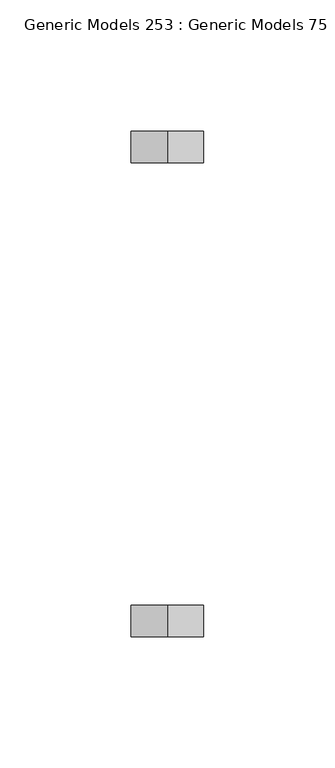
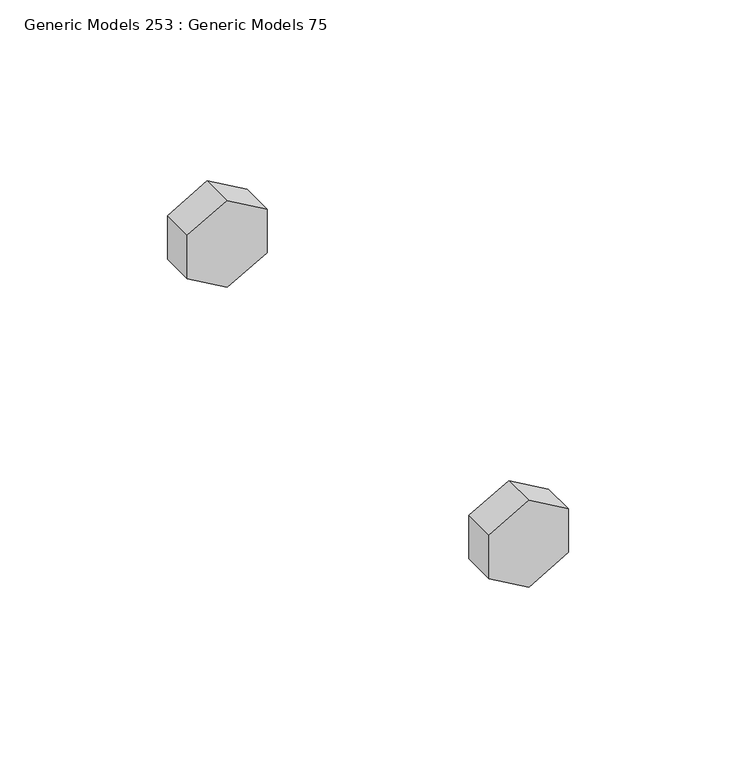
"""IFC4 building model written with IfcOpenShell, lengths in millimetres: proxy geometry, Generic Models 253 : Generic Models 75."""

from ifc_helpers import new_model, si_unit, frame, origin, place, context, project, spatial, polyline, outline, extrude, source, transform, mapped, element, save


def generic_models_253_generic_models_75_2b1a786a(model_context):
    return source(origin(), model_context, "Body", "SweptSolid", [
        extrude(outline(polyline([(269374.7462802, 31975.9942029), (269358.9097067, 31975.9942029), (269350.99142, 31989.7090778), (269358.9097067, 32003.4239528), (269374.7462802, 32003.4239528), (269382.664567, 31989.7090778), (269374.7462802, 31975.9942029)])), frame((0.0, 30858.4781612, 0.0), z_axis=(0.0, 1.0, 0.0), x_axis=(0.0, 0.0, 1.0)), (0.0, 0.0, 1.0), 11.90625),
        extrude(outline(polyline([(269374.7462802, 31975.9942029), (269358.9097067, 31975.9942029), (269350.99142, 31989.7090778), (269358.9097067, 32003.4239528), (269374.7462802, 32003.4239528), (269382.664567, 31989.7090778), (269374.7462802, 31975.9942029)])), frame((0.0, 30678.2969112, 0.0), z_axis=(0.0, 1.0, 0.0), x_axis=(0.0, 0.0, 1.0)), (0.0, 0.0, 1.0), 11.90625),
    ])


if __name__ == "__main__":
    model = new_model("IFC4")
    model_context = context("Model", 3, world=origin())
    ifc_project = project(units=[si_unit("LENGTHUNIT", "METRE", prefix="MILLI")], contexts=[model_context])
    site = spatial("IfcSite", under=ifc_project)
    building = spatial("IfcBuilding", under=site)
    placement = place(None, origin())
    generic_models_253_generic_models_75_shape = generic_models_253_generic_models_75_2b1a786a(model_context)
    element("IfcBuildingElementProxy", 1, Name="Generic Models 253 : Generic Models 75", ObjectType="Generic Models 253 : Generic Models 75", at=placement, inside=building, context=model_context, shape_type="MappedRepresentation", body=[
        mapped(generic_models_253_generic_models_75_shape, transform((0.0, 0.0, 0.0), x_axis=(1.0, 0.0, 0.0), y_axis=(0.0, 1.0, 0.0), z_axis=(0.0, 0.0, 1.0))),
    ])
    save(model, "model.ifc")

# Revit data of these elements
# Element 1 (IfcBuildingElementProxy, "Generic Models 253 : Generic Models 75")
#   Materials on its faces: "3/4\" GALV. THRU BOLTS"
# Materials
#   "3/4\" GALV. THRU BOLTS": class "Generic", colour RGB 105 69 171, transparency 0, Cost = 0
